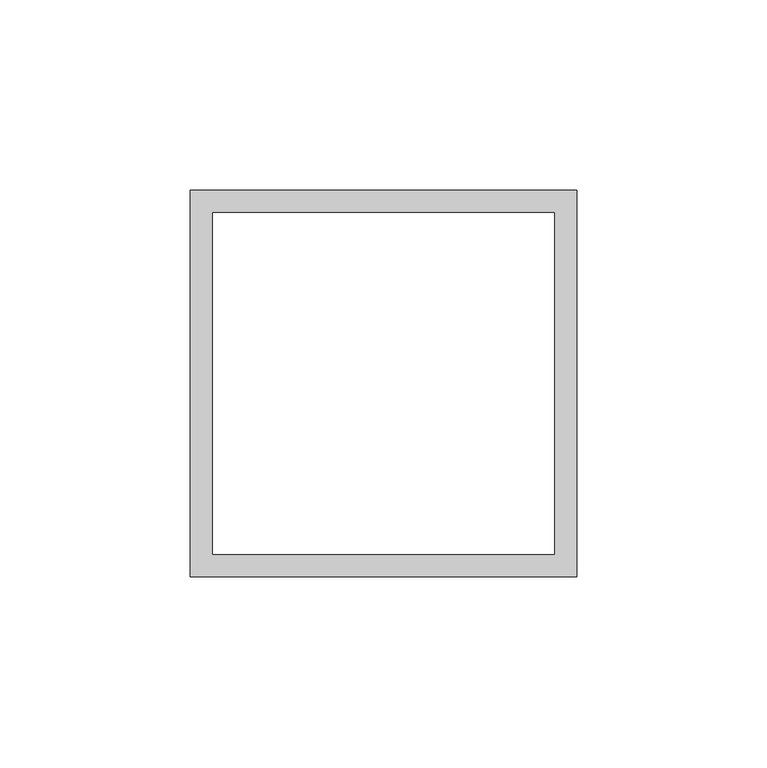
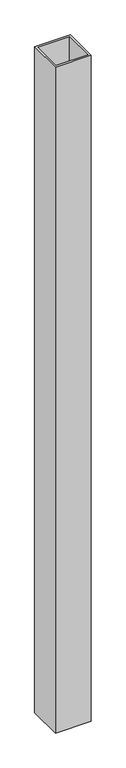
"""IFC4 building model written with IfcOpenShell, lengths in millimetres: proxy geometry, Generic Models 7:Generic Models 1:3:Generic Models 1:3 : Generic Models 7:Generic Models 1:305549:3:Generic Models 1:3:Generic Models 1:3 : Generic Models 7:Generic Models 1:305549:3 : Generic Models 7:Generic Models 1:3:Generic Models 1:3 : Generic Models 7:Generic Models 1:305549:301244:17 : Generic Models 7:Generic Models 1:3:Generic Models 1:3 : Generic Models 7:Generic Models 1:305549:3:Generic Models 1:3:Generic Models 1:3 : Generic Models 7:Generic Models 1:305549:3 : Generic Models 7:Generic Models 1:3:Generic Models 1:3 : Generic Models 7:Generic Models 1:305549:301244:308848."""

import ifcopenshell
import ifcopenshell.guid

model = None  # the IFC model being written
_history = None  # IfcOwnerHistory: only IFC2X3 demands one
_inside = {}  # id of a spatial element -> (the spatial element, [elements in it])
_under = {}  # id of a project, library or spatial element -> (it, [spatial elements below it])
_declared = {}  # id of a project -> (the project, [libraries it declares])
_typed = {}  # id of a type object -> (the type object, [elements of that type])
_made_of = {}  # id of a material, layer set ... -> (it, [elements and type objects made of it])


def new_model(schema):
    """Start an empty IFC model of exactly this schema.

    Asked for "IFC4X3", IfcOpenShell would pick the latest addendum, in which some entities
    have other attributes; the version numbers below select the first issue.
    IFC2X3 requires an IfcOwnerHistory on every rooted entity: one is made here for all.
    """
    global model, _history
    if schema == "IFC4X3":
        model = ifcopenshell.file(schema_version=(4, 3, 0, 0))
    else:
        model = ifcopenshell.file(schema=schema)
    _inside.clear()
    _under.clear()
    _declared.clear()
    _typed.clear()
    _made_of.clear()
    _history = None
    if model.schema == "IFC2X3":
        org = make("IfcOrganization", Name="unknown")
        user = make(
            "IfcPersonAndOrganization",
            ThePerson=make("IfcPerson", FamilyName="unknown"),
            TheOrganization=org,
        )
        app = make(
            "IfcApplication",
            ApplicationDeveloper=org,
            Version="unknown",
            ApplicationFullName="unknown",
            ApplicationIdentifier="unknown",
        )
        _history = make(
            "IfcOwnerHistory",
            OwningUser=user,
            OwningApplication=app,
            ChangeAction="ADDED",
            CreationDate=0,
        )
    return model


def make(cls, **values):
    """One entity of the class cls with the attributes given. An attribute that is None is left unset."""
    return model.create_entity(
        cls, **{name: value for name, value in values.items() if value is not None}
    )


def rooted(cls, **values):
    """An entity with a GlobalId (a new one), such as an element, a storey or a relation."""
    return make(cls, GlobalId=ifcopenshell.guid.new(), OwnerHistory=_history, **values)


def si_unit(unit_type, name, prefix=None):
    """IfcSIUnit, for example si_unit("LENGTHUNIT", "METRE", prefix="MILLI")."""
    return make("IfcSIUnit", UnitType=unit_type, Prefix=prefix, Name=name)


def assignment(units):
    """IfcUnitAssignment: the units of a project."""
    return None if units is None else make("IfcUnitAssignment", Units=units)


def point(xyz):
    """IfcCartesianPoint."""
    return None if xyz is None else make("IfcCartesianPoint", Coordinates=xyz)


def direction(xyz):
    """IfcDirection."""
    return None if xyz is None else make("IfcDirection", DirectionRatios=xyz)


def frame(location, z_axis=None, x_axis=None):
    """IfcAxis2Placement3D, a coordinate frame: its origin and axes. An axis left out is left unset."""
    return make(
        "IfcAxis2Placement3D",
        Location=point(location),
        Axis=direction(z_axis),
        RefDirection=direction(x_axis),
    )


def origin():
    """The frame at (0, 0, 0) with its axes left unset."""
    return frame((0.0, 0.0, 0.0))


def place(relative_to, where):
    """IfcLocalPlacement: puts the frame where relative to a parent placement (None: the world)."""
    return make(
        "IfcLocalPlacement", PlacementRelTo=relative_to, RelativePlacement=where
    )


def context(
    kind, dimensions, precision=None, world=None, true_north=None, identifier=None
):
    """IfcGeometricRepresentationContext, for example the 3D "Model" context."""
    return make(
        "IfcGeometricRepresentationContext",
        ContextIdentifier=identifier,
        ContextType=kind,
        CoordinateSpaceDimension=dimensions,
        Precision=precision,
        WorldCoordinateSystem=world,
        TrueNorth=true_north,
    )


def project(units=None, contexts=None):
    """IfcProject with its units and contexts."""
    return rooted(
        "IfcProject",
        Name="project",
        RepresentationContexts=contexts,
        UnitsInContext=assignment(units),
    )


def spatial(cls, under=None, at=None, **own):
    """A site, building, storey or space (cls), placed at a placement, below another one or the project."""
    s = rooted(cls, ObjectPlacement=at, **own)
    if under is not None:
        _under.setdefault(under.id(), (under, []))[1].append(s)
    return s


def polyline(points):
    """IfcPolyline through the points."""
    return make("IfcPolyline", Points=[point(p) for p in points])


def outline(outer, holes=None, kind="AREA"):
    """IfcArbitraryClosedProfileDef: a profile drawn as a closed curve; with holes, ...WithVoids."""
    if holes is None:
        return make("IfcArbitraryClosedProfileDef", ProfileType=kind, OuterCurve=outer)
    return make(
        "IfcArbitraryProfileDefWithVoids",
        ProfileType=kind,
        OuterCurve=outer,
        InnerCurves=holes,
    )


def extrude(swept, where, along, depth):
    """IfcExtrudedAreaSolid: the profile swept, set in the frame where, extruded along a direction by depth."""
    return make(
        "IfcExtrudedAreaSolid",
        SweptArea=swept,
        Position=where,
        ExtrudedDirection=direction(along),
        Depth=depth,
    )


def shape(context_of_items, identifier, shape_type, items):
    """IfcShapeRepresentation: the items that make up one representation, for example the "Body"."""
    return make(
        "IfcShapeRepresentation",
        ContextOfItems=context_of_items,
        RepresentationIdentifier=identifier,
        RepresentationType=shape_type,
        Items=items,
    )


def source(mapping_origin, context_of_items, identifier, shape_type, items):
    """IfcRepresentationMap: a shape defined once, which mapped items show again and again."""
    return make(
        "IfcRepresentationMap",
        MappingOrigin=mapping_origin,
        MappedRepresentation=shape(context_of_items, identifier, shape_type, items),
    )


def transform(
    local_origin,
    x_axis=None,
    y_axis=None,
    z_axis=None,
    scale=None,
    scale2=None,
    scale3=None,
    uniform=True,
):
    """IfcCartesianTransformationOperator3D, or its non-uniform kind. x_axis, y_axis, z_axis: its Axis1, 2, 3."""
    if uniform:
        return make(
            "IfcCartesianTransformationOperator3D",
            Axis1=direction(x_axis),
            Axis2=direction(y_axis),
            LocalOrigin=point(local_origin),
            Scale=scale,
            Axis3=direction(z_axis),
        )
    return make(
        "IfcCartesianTransformationOperator3DnonUniform",
        Axis1=direction(x_axis),
        Axis2=direction(y_axis),
        LocalOrigin=point(local_origin),
        Scale=scale,
        Axis3=direction(z_axis),
        Scale2=scale2,
        Scale3=scale3,
    )


def mapped(mapping_source, mapping_target):
    """IfcMappedItem: shows the shape of a source again, moved by a transform."""
    return make(
        "IfcMappedItem", MappingSource=mapping_source, MappingTarget=mapping_target
    )


def made_of(thing, what):
    """Note that an element or type object is made of a material, layer set ...; save() writes the relation."""
    if what is not None:
        _made_of.setdefault(what.id(), (what, []))[1].append(thing)
    return thing


def element(
    cls,
    number,
    at=None,
    inside=None,
    cuts=None,
    type_object=None,
    material=None,
    context=None,
    identifier="Body",
    shape_type=None,
    held_by="IfcProductDefinitionShape",
    body=None,
    shapes=None,
    **own,
):
    """One element of the class cls, such as IfcWall. Its Tag is "e" and its number.

    at: its placement. inside: the storey or other place that contains it. cuts: it is an
    opening in that element (IfcRelVoidsElement). A single representation is given by context,
    identifier, shape_type and body (its items); several are given by shapes. held_by: the class
    of the entity that holds the representations. save() writes the other relations.
    """
    e = rooted(cls, Tag="e%d" % number, ObjectPlacement=at, **own)
    if body is not None:
        shapes = [shape(context, identifier, shape_type, body)]
    if shapes is not None:
        e.Representation = make(held_by, Representations=shapes)
    if inside is not None:
        _inside.setdefault(inside.id(), (inside, []))[1].append(e)
    if cuts is not None:
        rooted(
            "IfcRelVoidsElement", RelatingBuildingElement=cuts, RelatedOpeningElement=e
        )
    if type_object is not None:
        _typed.setdefault(type_object.id(), (type_object, []))[1].append(e)
    return made_of(e, material)


def aggregate(whole, parts):
    """IfcRelAggregates: a whole, such as a stair, and the parts it consists of."""
    return rooted("IfcRelAggregates", RelatingObject=whole, RelatedObjects=parts)


def save(model, path):
    """Write the relations noted so far, then the file.

    IfcRelAggregates (storeys below a building ...), IfcRelContainedInSpatialStructure (elements
    in a storey), IfcRelDefinesByType, IfcRelAssociatesMaterial and IfcRelDeclares: one each for
    every whole, place, type object, material and project.
    """
    for whole, parts in _under.values():
        aggregate(whole, parts)
    for where, things in _inside.values():
        rooted(
            "IfcRelContainedInSpatialStructure",
            RelatedElements=things,
            RelatingStructure=where,
        )
    for kind, things in _typed.values():
        rooted("IfcRelDefinesByType", RelatedObjects=things, RelatingType=kind)
    for what, things in _made_of.values():
        rooted("IfcRelAssociatesMaterial", RelatedObjects=things, RelatingMaterial=what)
    for by, libraries in _declared.values():
        rooted("IfcRelDeclares", RelatingContext=by, RelatedDefinitions=libraries)
    model.write(path)


def generic_models_e3ee71aa(model_context):
    return source(origin(), model_context, "Body", "SweptSolid", [
        extrude(outline(polyline([(560619.6617239, -578797.4842061), (560619.6617239, -578899.0842061), (560518.0617239, -578899.0842061), (560518.0617239, -578797.4842061), (560619.6617239, -578797.4842061)]), holes=[polyline([(560613.7435239, -578893.1660061), (560613.7435239, -578803.4024061), (560523.9799239, -578803.4024061), (560523.9799239, -578893.1660061), (560613.7435239, -578893.1660061)])]), frame((0.0, 0.0, 4133.81326), z_axis=(0.0, 0.0, 1.0), x_axis=(1.0, 0.0, 0.0)), (0.0, 0.0, 1.0), 2000.28674),
    ])


if __name__ == "__main__":
    model = new_model("IFC4")
    model_context = context("Model", 3, world=origin())
    ifc_project = project(units=[si_unit("LENGTHUNIT", "METRE", prefix="MILLI")], contexts=[model_context])
    site = spatial("IfcSite", under=ifc_project)
    building = spatial("IfcBuilding", under=site)
    placement = place(None, origin())
    generic_models_shape = generic_models_e3ee71aa(model_context)
    element("IfcBuildingElementProxy", 1, Name="Generic Models 7:Generic Models 1:3:Generic Models 1:3 : Generic Models 7:Generic Models 1:305549:3:Generic Models 1:3:Generic Models 1:3 : Generic Models 7:Generic Models 1:305549:3 : Generic Models 7:Generic Models 1:3:Generic Models 1:3 : Generic Models 7:Generic Models 1:305549:301244:17 : Generic Models 7:Generic Models 1:3:Generic Models 1:3 : Generic Models 7:Generic Models 1:305549:3:Generic Models 1:3:Generic Models 1:3 : Generic Models 7:Generic Models 1:305549:3 : Generic Models 7:Generic Models 1:3:Generic Models 1:3 : Generic Models 7:Generic Models 1:305549:301244:308848", ObjectType="Generic Models 7:Generic Models 1:3:Generic Models 1:3 : Generic Models 7:Generic Models 1:305549:3:Generic Models 1:3:Generic Models 1:3 : Generic Models 7:Generic Models 1:305549:3 : Generic Models 7:Generic Models 1:3:Generic Models 1:3 : Generic Models 7:Generic Models 1:305549:301244:17 : Generic Models 7:Generic Models 1:3:Generic Models 1:3 : Generic Models 7:Generic Models 1:305549:3:Generic Models 1:3:Generic Models 1:3 : Generic Models 7:Generic Models 1:305549:3 : Generic Models 7:Generic Models 1:3:Generic Models 1:3 : Generic Models 7:Generic Models 1:305549:301244:308848", at=placement, inside=building, context=model_context, shape_type="MappedRepresentation", body=[
        mapped(generic_models_shape, transform((0.0, 0.0, 0.0), x_axis=(1.0, 0.0, 0.0), y_axis=(0.0, 1.0, 0.0), z_axis=(0.0, 0.0, 1.0))),
    ])
    save(model, "model.ifc")

# Revit data of these elements
# Type "Generic Models 7:Generic Models 1:3:Generic Models 1:3 : Generic Models 7:Generic Models 1:305549:3:Generic Models 1:3:Generic Models 1:3 : Generic Models 7:Generic Models 1:305549:3 : Generic Models 7:Generic Models 1:3:Generic Models 1:3 : Generic Models 7:Generic Models 1:305549:301244:17 : Generic Models 7:Generic Models 1:3:Generic Models 1:3 : Generic Models 7:Generic Models 1:305549:3:Generic Models 1:3:Generic Models 1:3 : Generic Models 7:Generic Models 1:305549:3 : Generic Models 7:Generic Models 1:3:Generic Models 1:3 : Generic Models 7:Generic Models 1:305549:301244:308848"
#   NameOverride = "Generic Models 7:Generic Models 1:3:Generic Models 1:3 : Generic Models 7:Generic Models 1:305549:3:Generic Models 1:3:Generic Models 1:3 : Generic Models 7:Generic Models 1:305549:3 : Generic Models 7:Generic Models 1:3:Generic Models 1:3 : Generic Models 7:Generic Models 1:305549:301244:308848"
#   ObjectTypeOverride = "Generic Models 1:3:Generic Models 1:3 : Generic Models 7:Generic Models 1:305549:3 : Generic Models 7:Generic Models 1:3:Generic Models 1:3 : Generic Models 7:Generic Models 1:305549:301244"
#   Reference = "Generic Models 1"
#   Tag = "308848"
# Element 1 (IfcBuildingElementProxy, "Generic Models 7:Generic Models 1:3:Generic Models 1:3 : Generic Models 7:Generic Models 1:305549:3:Generic Models 1:3:Generic Models 1:3 : Generic Models 7:Generic Models 1:305549:3 : Generic Models 7:Generic Models 1:3:Generic Models 1:3 : Generic Models 7:Generic Models 1:305549:301244:17 : Generic Models 7:Generic Models 1:3:Generic Models 1:3 : Generic Models 7:Generic Models 1:305549:3:Generic Models 1:3:Generic Models 1:3 : Generic Models 7:Generic Models 1:305549:3 : Generic Models 7:Generic Models 1:3:Generic Models 1:3 : Generic Models 7:Generic Models 1:305549:301244:308848")
#   Materials on its faces: "STRUCTURAL STEEL - SEE STRUCT. DWGS"
# Materials
#   "STRUCTURAL STEEL - SEE STRUCT. DWGS": class "Metal", colour RGB 189 187 185, transparency 0, Description = "Structural steel 50ksi", Cost = 0
